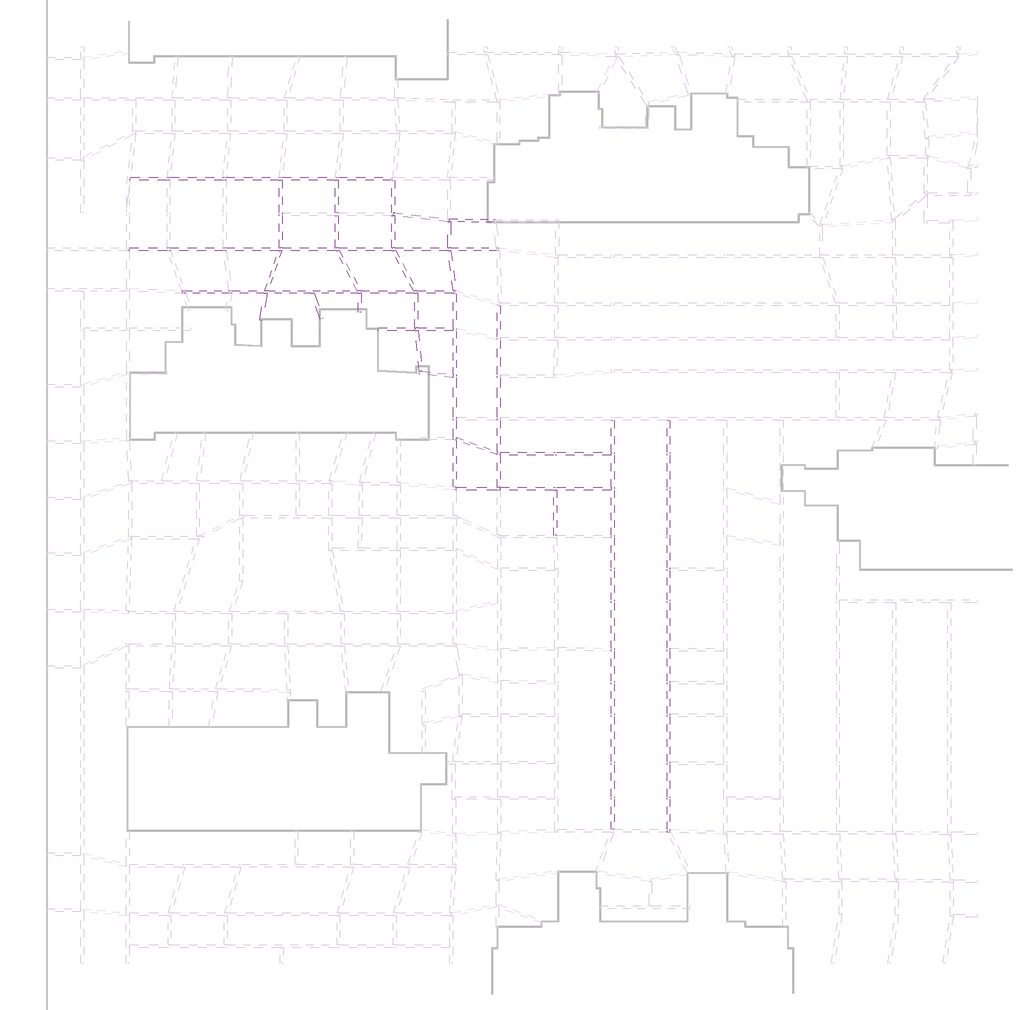
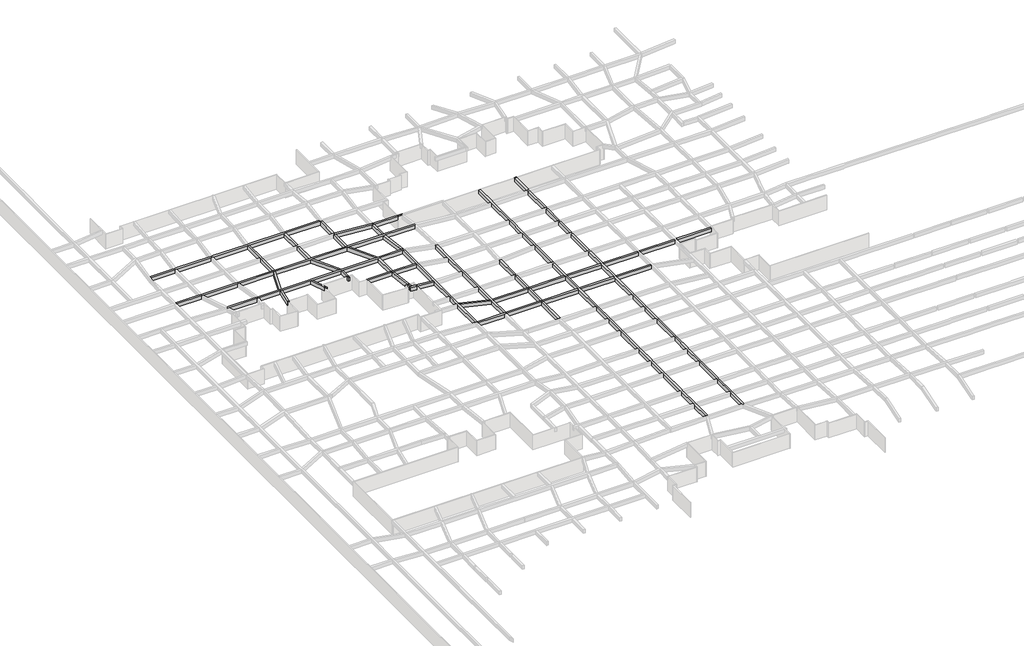
# One storey, part 27 of 45: 32 beams.
"""IFC4 building model written with IfcOpenShell, lengths in millimetres."""

from ifc_helpers import new_model, si_unit, frame, origin, place, context, project, spatial, polyline, outline, extrude, faceted_brep, element, save

model = new_model("IFC4")

# Units and contexts
model_context = context("Model", 3, world=origin())
ifc_project = project(units=[si_unit("LENGTHUNIT", "METRE", prefix="MILLI")], contexts=[model_context])

# Site, building, storey
site = spatial("IfcSite", under=ifc_project)
building = spatial("IfcBuilding", under=site)
storey = spatial("IfcBuildingStorey", under=building, Name="户型图", Elevation=0.0)

# Beams
placement = place(None, origin())
element("IfcBeam", 1, ObjectType="混凝土 - 矩形梁 : KL_beam", at=placement, inside=storey, context=model_context, shape_type="Brep", body=[
    faceted_brep([(-76574.0592951, 55456.2114264, 3300.0), (-76574.0592951, 55456.2114264, 2500.0), (-76974.0592951, 55456.2114264, 2500.0), (-76974.0592951, 55456.2114264, 3300.0), (-76574.0592951, 28384.5858537, 3300.0), (-76974.0592951, 28384.5858537, 3300.0), (-76974.0592951, 28384.5858537, 2500.0), (-76574.0592951, 28384.5858537, 2500.0), (-76974.0592951, 50864.7430833, 3300.0), (-76974.0592951, 50464.7430833, 3300.0), (-76974.0592951, 44242.2010773, 3300.0), (-76974.0592951, 43842.2010773, 3300.0), (-76974.0592951, 39470.5101546, 3300.0), (-76974.0592951, 39070.5101546, 3300.0), (-76974.0592951, 34954.5846853, 3300.0), (-76974.0592951, 34553.0567503, 3300.0), (-76574.0592951, 34571.3370449, 3300.0), (-76574.0592951, 34971.3370449, 3300.0), (-76574.0592951, 39070.5101546, 3300.0), (-76574.0592951, 39470.5101546, 3300.0), (-76574.0592951, 43842.2010773, 3300.0), (-76574.0592951, 44242.2010773, 3300.0), (-76574.0592951, 50450.070339, 3300.0), (-76574.0592951, 50850.070339, 3300.0), (-76974.0592951, 50864.7430833, 2500.0), (-76974.0592951, 50464.7430833, 2500.0), (-76974.0592951, 44242.2010773, 2500.0), (-76974.0592951, 43842.2010773, 2500.0), (-76974.0592951, 39470.5101546, 2500.0), (-76974.0592951, 39070.5101546, 2500.0), (-76974.0592951, 34954.5846853, 2500.0), (-76974.0592951, 34553.0567503, 2500.0), (-76574.0592951, 50850.070339, 2500.0), (-76574.0592951, 50450.070339, 2500.0), (-76574.0592951, 44242.2010773, 2500.0), (-76574.0592951, 43842.2010773, 2500.0), (-76574.0592951, 39470.5101546, 2500.0), (-76574.0592951, 39070.5101546, 2500.0), (-76574.0592951, 34971.3370449, 2500.0), (-76574.0592951, 34571.3370449, 2500.0)], [[[0, 1, 2, 3]], [[4, 5, 6, 7]], [[0, 3, 8, 9, 10, 11, 12, 13, 14, 15, 5, 4, 16, 17, 18, 19, 20, 21, 22, 23]], [[3, 2, 24, 25, 26, 27, 28, 29, 30, 31, 6, 5, 15, 14, 13, 12, 11, 10, 9, 8]], [[2, 1, 32, 33, 34, 35, 36, 37, 38, 39, 7, 6, 31, 30, 29, 28, 27, 26, 25, 24]], [[1, 0, 23, 22, 21, 20, 19, 18, 17, 16, 4, 7, 39, 38, 37, 36, 35, 34, 33, 32]]]),
    faceted_brep([(-76574.0592951, 27984.5858537, 3300.0), (-76974.0592951, 27984.5858537, 3300.0), (-76974.0592951, 23571.3370449, 3300.0), (-76974.0592951, 23171.3370449, 3300.0), (-76974.0592951, 18720.4464741, 3300.0), (-76974.0592951, 18320.4464741, 3300.0), (-76974.0592951, 12100.217385, 3300.0), (-76974.0592951, 11700.217385, 3300.0), (-76974.0592951, 7600.318112, 3300.0), (-76974.0592951, 7200.318112, 3300.0), (-76974.0592951, 3119.5822838, 3300.0), (-76974.0592951, 2719.5822838, 3300.0), (-76974.0592951, -3547.9984335, 3300.0), (-76974.0592951, -3948.0593648, 3300.0), (-76974.0592951, -8106.533538, 3300.0), (-76974.0592951, -8506.533538, 3300.0), (-76974.0592951, -12606.533538, 3300.0), (-76974.0592951, -13006.533538, 3300.0), (-76974.0592951, -19266.2432363, 3300.0), (-76974.0592951, -19666.2432363, 3300.0), (-76974.0592951, -24066.2432363, 3300.0), (-76974.0592951, -24466.2432363, 3300.0), (-76974.0592951, -28597.0413366, 3300.0), (-76574.0592951, -28597.0413366, 3300.0), (-76574.0592951, -24466.2432363, 3300.0), (-76574.0592951, -24066.2432363, 3300.0), (-76574.0592951, -19666.2432363, 3300.0), (-76574.0592951, -19266.2432363, 3300.0), (-76574.0592951, -13006.533538, 3300.0), (-76574.0592951, -12606.533538, 3300.0), (-76574.0592951, -8506.533538, 3300.0), (-76574.0592951, -8106.533538, 3300.0), (-76574.0592951, -3951.5199121, 3300.0), (-76574.0592951, -3551.5199121, 3300.0), (-76574.0592951, 2719.5822838, 3300.0), (-76574.0592951, 3119.5822838, 3300.0), (-76574.0592951, 7200.318112, 3300.0), (-76574.0592951, 7600.318112, 3300.0), (-76574.0592951, 11700.217385, 3300.0), (-76574.0592951, 12100.217385, 3300.0), (-76574.0592951, 18320.4464741, 3300.0), (-76574.0592951, 18720.4464741, 3300.0), (-76574.0592951, 23171.3370449, 3300.0), (-76574.0592951, 23571.3370449, 3300.0), (-76974.0592951, 27984.5858537, 2500.0), (-76974.0592951, 23571.3370449, 2500.0), (-76974.0592951, 23171.3370449, 2500.0), (-76974.0592951, 18720.4464741, 2500.0), (-76974.0592951, 18320.4464741, 2500.0), (-76974.0592951, 12100.217385, 2500.0), (-76974.0592951, 11700.217385, 2500.0), (-76974.0592951, 7600.318112, 2500.0), (-76974.0592951, 7200.318112, 2500.0), (-76974.0592951, 3119.5822838, 2500.0), (-76974.0592951, 2719.5822838, 2500.0), (-76974.0592951, -3547.9984335, 2500.0), (-76974.0592951, -3948.0593648, 2500.0), (-76974.0592951, -8106.533538, 2500.0), (-76974.0592951, -8506.533538, 2500.0), (-76974.0592951, -12606.533538, 2500.0), (-76974.0592951, -13006.533538, 2500.0), (-76974.0592951, -19266.2432363, 2500.0), (-76974.0592951, -19666.2432363, 2500.0), (-76974.0592951, -24066.2432363, 2500.0), (-76974.0592951, -24466.2432363, 2500.0), (-76974.0592951, -28597.0413366, 2500.0), (-76574.0592951, 27984.5858537, 2500.0), (-76574.0592951, 23571.3370449, 2500.0), (-76574.0592951, 23171.3370449, 2500.0), (-76574.0592951, 18720.4464741, 2500.0), (-76574.0592951, 18320.4464741, 2500.0), (-76574.0592951, 12100.217385, 2500.0), (-76574.0592951, 11700.217385, 2500.0), (-76574.0592951, 7600.318112, 2500.0), (-76574.0592951, 7200.318112, 2500.0), (-76574.0592951, 3119.5822838, 2500.0), (-76574.0592951, 2719.5822838, 2500.0), (-76574.0592951, -3551.5199121, 2500.0), (-76574.0592951, -3951.5199121, 2500.0), (-76574.0592951, -8106.533538, 2500.0), (-76574.0592951, -8506.533538, 2500.0), (-76574.0592951, -12606.533538, 2500.0), (-76574.0592951, -13006.533538, 2500.0), (-76574.0592951, -19266.2432363, 2500.0), (-76574.0592951, -19666.2432363, 2500.0), (-76574.0592951, -24066.2432363, 2500.0), (-76574.0592951, -24466.2432363, 2500.0), (-76574.0592951, -28597.0413366, 2500.0)], [[[0, 1, 2, 3, 4, 5, 6, 7, 8, 9, 10, 11, 12, 13, 14, 15, 16, 17, 18, 19, 20, 21, 22, 23, 24, 25, 26, 27, 28, 29, 30, 31, 32, 33, 34, 35, 36, 37, 38, 39, 40, 41, 42, 43]], [[1, 44, 45, 46, 47, 48, 49, 50, 51, 52, 53, 54, 55, 56, 57, 58, 59, 60, 61, 62, 63, 64, 65, 22, 21, 20, 19, 18, 17, 16, 15, 14, 13, 12, 11, 10, 9, 8, 7, 6, 5, 4, 3, 2]], [[44, 66, 67, 68, 69, 70, 71, 72, 73, 74, 75, 76, 77, 78, 79, 80, 81, 82, 83, 84, 85, 86, 87, 65, 64, 63, 62, 61, 60, 59, 58, 57, 56, 55, 54, 53, 52, 51, 50, 49, 48, 47, 46, 45]], [[66, 0, 43, 42, 41, 40, 39, 38, 37, 36, 35, 34, 33, 32, 31, 30, 29, 28, 27, 26, 25, 24, 23, 87, 86, 85, 84, 83, 82, 81, 80, 79, 78, 77, 76, 75, 74, 73, 72, 71, 70, 69, 68, 67]], [[1, 0, 66, 44]], [[23, 22, 65, 87]]]),
])
element("IfcBeam", 2, ObjectType="混凝土 - 矩形梁 : KL_beam", at=placement, inside=storey, context=model_context, shape_type="Brep", body=[
    faceted_brep([(-68859.410716, 55506.2431184, 3300.0), (-68859.410716, 55506.2431184, 2500.0), (-69259.410716, 55506.2431184, 2500.0), (-69259.410716, 55506.2431184, 3300.0), (-68859.410716, 50850.070339, 3300.0), (-69259.410716, 50850.070339, 3300.0), (-69259.410716, 50850.070339, 2500.0), (-68859.410716, 50850.070339, 2500.0)], [[[0, 1, 2, 3]], [[4, 5, 6, 7]], [[0, 3, 5, 4]], [[3, 2, 6, 5]], [[2, 1, 7, 6]], [[1, 0, 4, 7]]]),
    faceted_brep([(-68859.410716, 27984.5858537, 3300.0), (-69259.410716, 27984.5858537, 3300.0), (-69259.410716, 23571.3370449, 3300.0), (-69259.410716, 23171.3370449, 3300.0), (-69259.410716, 18720.4464741, 3300.0), (-69259.410716, 18320.4464741, 3300.0), (-69259.410716, 12100.217385, 3300.0), (-69259.410716, 11700.217385, 3300.0), (-69259.410716, 7600.318112, 3300.0), (-69259.410716, 7200.318112, 3300.0), (-69259.410716, 3119.5822838, 3300.0), (-69259.410716, 2719.5822838, 3300.0), (-69259.410716, -3551.5199121, 3300.0), (-69259.410716, -3951.5199121, 3300.0), (-69259.410716, -8106.533538, 3300.0), (-69259.410716, -8506.533538, 3300.0), (-69259.410716, -12606.533538, 3300.0), (-69259.410716, -13006.533538, 3300.0), (-69259.410716, -19266.2432363, 3300.0), (-69259.410716, -19666.2432363, 3300.0), (-69259.410716, -24066.2432363, 3300.0), (-69259.410716, -24466.2432363, 3300.0), (-69259.410716, -28597.0413366, 3300.0), (-69259.410716, -28997.0413366, 3300.0), (-69183.9947177, -28997.0413366, 3300.0), (-69062.8285047, -28997.0413366, 3300.0), (-68859.410716, -28997.0413366, 3300.0), (-68859.410716, -28603.762064, 3300.0), (-68859.410716, -24466.2432363, 3300.0), (-68859.410716, -24066.2432363, 3300.0), (-68859.410716, -19666.2432363, 3300.0), (-68859.410716, -19266.2432363, 3300.0), (-68859.410716, -13006.533538, 3300.0), (-68859.410716, -12606.533538, 3300.0), (-68859.410716, -8506.533538, 3300.0), (-68859.410716, -8106.533538, 3300.0), (-68859.410716, -3951.5199121, 3300.0), (-68859.410716, -3551.5199121, 3300.0), (-68859.410716, 2719.5822838, 3300.0), (-68859.410716, 3119.5822838, 3300.0), (-68859.410716, 7200.318112, 3300.0), (-68859.410716, 7600.318112, 3300.0), (-68859.410716, 11700.217385, 3300.0), (-68859.410716, 12100.217385, 3300.0), (-68859.410716, 18320.4464741, 3300.0), (-68859.410716, 18720.4464741, 3300.0), (-68859.410716, 23171.3370449, 3300.0), (-68859.410716, 23571.3370449, 3300.0), (-69259.410716, 27984.5858537, 2500.0), (-69259.410716, 23571.3370449, 2500.0), (-69259.410716, 23171.3370449, 2500.0), (-69259.410716, 18720.4464741, 2500.0), (-69259.410716, 18320.4464741, 2500.0), (-69259.410716, 12100.217385, 2500.0), (-69259.410716, 11700.217385, 2500.0), (-69259.410716, 7600.318112, 2500.0), (-69259.410716, 7200.318112, 2500.0), (-69259.410716, 3119.5822838, 2500.0), (-69259.410716, 2719.5822838, 2500.0), (-69259.410716, -3551.5199121, 2500.0), (-69259.410716, -3951.5199121, 2500.0), (-69259.410716, -8106.533538, 2500.0), (-69259.410716, -8506.533538, 2500.0), (-69259.410716, -12606.533538, 2500.0), (-69259.410716, -13006.533538, 2500.0), (-69259.410716, -19266.2432363, 2500.0), (-69259.410716, -19666.2432363, 2500.0), (-69259.410716, -24066.2432363, 2500.0), (-69259.410716, -24466.2432363, 2500.0), (-69259.410716, -28597.0413366, 2500.0), (-69259.410716, -28997.0413366, 2500.0), (-68859.410716, 27984.5858537, 2500.0), (-68859.410716, 23571.3370449, 2500.0), (-68859.410716, 23171.3370449, 2500.0), (-68859.410716, 18720.4464741, 2500.0), (-68859.410716, 18320.4464741, 2500.0), (-68859.410716, 12100.217385, 2500.0), (-68859.410716, 11700.217385, 2500.0), (-68859.410716, 7600.318112, 2500.0), (-68859.410716, 7200.318112, 2500.0), (-68859.410716, 3119.5822838, 2500.0), (-68859.410716, 2719.5822838, 2500.0), (-68859.410716, -3551.5199121, 2500.0), (-68859.410716, -3951.5199121, 2500.0), (-68859.410716, -8106.533538, 2500.0), (-68859.410716, -8506.533538, 2500.0), (-68859.410716, -12606.533538, 2500.0), (-68859.410716, -13006.533538, 2500.0), (-68859.410716, -19266.2432363, 2500.0), (-68859.410716, -19666.2432363, 2500.0), (-68859.410716, -24066.2432363, 2500.0), (-68859.410716, -24466.2432363, 2500.0), (-68859.410716, -28603.762064, 2500.0), (-68859.410716, -28997.0413366, 2500.0), (-69062.8285047, -28997.0413366, 2500.0), (-69183.9947177, -28997.0413366, 2500.0)], [[[0, 1, 2, 3, 4, 5, 6, 7, 8, 9, 10, 11, 12, 13, 14, 15, 16, 17, 18, 19, 20, 21, 22, 23, 24, 25, 26, 27, 28, 29, 30, 31, 32, 33, 34, 35, 36, 37, 38, 39, 40, 41, 42, 43, 44, 45, 46, 47]], [[1, 48, 49, 50, 51, 52, 53, 54, 55, 56, 57, 58, 59, 60, 61, 62, 63, 64, 65, 66, 67, 68, 69, 70, 23, 22, 21, 20, 19, 18, 17, 16, 15, 14, 13, 12, 11, 10, 9, 8, 7, 6, 5, 4, 3, 2]], [[48, 71, 72, 73, 74, 75, 76, 77, 78, 79, 80, 81, 82, 83, 84, 85, 86, 87, 88, 89, 90, 91, 92, 93, 94, 95, 70, 69, 68, 67, 66, 65, 64, 63, 62, 61, 60, 59, 58, 57, 56, 55, 54, 53, 52, 51, 50, 49]], [[71, 0, 47, 46, 45, 44, 43, 42, 41, 40, 39, 38, 37, 36, 35, 34, 33, 32, 31, 30, 29, 28, 27, 26, 93, 92, 91, 90, 89, 88, 87, 86, 85, 84, 83, 82, 81, 80, 79, 78, 77, 76, 75, 74, 73, 72]], [[1, 0, 71, 48]], [[26, 25, 24, 23, 70, 95, 94, 93]]]),
    faceted_brep([(-68859.410716, 28384.5858537, 3300.0), (-69259.410716, 28384.5858537, 3300.0), (-69259.410716, 28384.5858537, 2500.0), (-68859.410716, 28384.5858537, 2500.0), (-68859.410716, 34571.3370449, 3300.0), (-69259.410716, 34571.3370449, 3300.0), (-69259.410716, 34571.3370449, 2500.0), (-68859.410716, 34571.3370449, 2500.0)], [[[0, 1, 2, 3]], [[1, 0, 4, 5]], [[2, 1, 5, 6]], [[3, 2, 6, 7]], [[0, 3, 7, 4]], [[5, 4, 7, 6]]]),
    faceted_brep([(-68859.410716, 34971.3370449, 3300.0), (-69259.410716, 34971.3370449, 3300.0), (-69259.410716, 34971.3370449, 2500.0), (-68859.410716, 34971.3370449, 2500.0), (-68859.410716, 39070.5101546, 3300.0), (-69259.410716, 39070.5101546, 3300.0), (-69259.410716, 39070.5101546, 2500.0), (-68859.410716, 39070.5101546, 2500.0)], [[[0, 1, 2, 3]], [[1, 0, 4, 5]], [[2, 1, 5, 6]], [[3, 2, 6, 7]], [[0, 3, 7, 4]], [[5, 4, 7, 6]]]),
    faceted_brep([(-68859.410716, 39470.5101546, 3300.0), (-69259.410716, 39470.5101546, 3300.0), (-69259.410716, 39470.5101546, 2500.0), (-68859.410716, 39470.5101546, 2500.0), (-68859.410716, 43842.2010773, 3300.0), (-69259.410716, 43842.2010773, 3300.0), (-69259.410716, 43842.2010773, 2500.0), (-68859.410716, 43842.2010773, 2500.0)], [[[0, 1, 2, 3]], [[1, 0, 4, 5]], [[2, 1, 5, 6]], [[3, 2, 6, 7]], [[0, 3, 7, 4]], [[5, 4, 7, 6]]]),
    faceted_brep([(-68859.410716, 44242.2010773, 3300.0), (-69259.410716, 44242.2010773, 3300.0), (-69259.410716, 44242.2010773, 2500.0), (-68859.410716, 44242.2010773, 2500.0), (-68859.410716, 50450.070339, 3300.0), (-69259.410716, 50450.070339, 3300.0), (-69259.410716, 50450.070339, 2500.0), (-68859.410716, 50450.070339, 2500.0)], [[[0, 1, 2, 3]], [[1, 0, 4, 5]], [[2, 1, 5, 6]], [[3, 2, 6, 7]], [[0, 3, 7, 4]], [[5, 4, 7, 6]]]),
])
element("IfcBeam", 3, ObjectType="混凝土 - 矩形梁 : KL_beam", at=placement, inside=storey, context=model_context, shape_type="Brep", body=[
    faceted_brep([(-107354.1744669, 61170.3096597, 3300.0), (-107354.1744669, 61570.3096597, 3300.0), (-114692.5916069, 61570.3096597, 3300.0), (-115094.7622577, 61570.3096597, 3300.0), (-122492.6084803, 61570.3096597, 3300.0), (-122894.779131, 61570.3096597, 3300.0), (-130266.1701137, 61570.3096597, 3300.0), (-130292.5916069, 61570.3096597, 3300.0), (-130694.7622577, 61570.3096597, 3300.0), (-137992.6084803, 61570.3096597, 3300.0), (-138394.779131, 61570.3096597, 3300.0), (-143507.3765183, 61570.3096597, 3300.0), (-143556.4903427, 61170.3096597, 3300.0), (-138430.1531976, 61170.3096597, 3300.0), (-138030.1531976, 61170.3096597, 3300.0), (-130666.1701137, 61170.3096597, 3300.0), (-130266.1701137, 61170.3096597, 3300.0), (-122902.1870297, 61170.3096597, 3300.0), (-122502.1870297, 61170.3096597, 3300.0), (-115128.2029549, 61170.3096597, 3300.0), (-114728.2029549, 61170.3096597, 3300.0), (-107354.1744669, 61170.3096597, 2500.0), (-143556.4903427, 61170.3096597, 2500.0), (-138430.1531976, 61170.3096597, 2500.0), (-138030.1531976, 61170.3096597, 2500.0), (-130666.1701137, 61170.3096597, 2500.0), (-130266.1701137, 61170.3096597, 2500.0), (-122902.1870297, 61170.3096597, 2500.0), (-122502.1870297, 61170.3096597, 2500.0), (-115128.2029549, 61170.3096597, 2500.0), (-114728.2029549, 61170.3096597, 2500.0), (-107354.1744669, 61570.3096597, 2500.0), (-143507.3765183, 61570.3096597, 2500.0), (-138394.779131, 61570.3096597, 2500.0), (-137992.6084803, 61570.3096597, 2500.0), (-130694.7622577, 61570.3096597, 2500.0), (-130292.5916069, 61570.3096597, 2500.0), (-130266.1701137, 61570.3096597, 2500.0), (-122894.779131, 61570.3096597, 2500.0), (-122492.6084803, 61570.3096597, 2500.0), (-115094.7622577, 61570.3096597, 2500.0), (-114692.5916069, 61570.3096597, 2500.0)], [[[0, 1, 2, 3, 4, 5, 6, 7, 8, 9, 10, 11, 12, 13, 14, 15, 16, 17, 18, 19, 20]], [[21, 0, 20, 19, 18, 17, 16, 15, 14, 13, 12, 22, 23, 24, 25, 26, 27, 28, 29, 30]], [[31, 21, 30, 29, 28, 27, 26, 25, 24, 23, 22, 32, 33, 34, 35, 36, 37, 38, 39, 40, 41]], [[1, 31, 41, 40, 39, 38, 37, 36, 35, 34, 33, 32, 11, 10, 9, 8, 7, 6, 5, 4, 3, 2]], [[1, 0, 21, 31]], [[12, 11, 32, 22]]]),
])
element("IfcBeam", 4, ObjectType="混凝土 - 矩形梁 : KL_beam", at=placement, inside=storey, context=model_context, shape_type="SweptSolid", body=[
    extrude(outline(polyline([(-106954.1744669, 56704.7417755), (-107354.1744669, 56704.7417755), (-107354.1744669, 61170.3096597), (-106954.1744669, 61170.3096597), (-106954.1744669, 56704.7417755)])), frame((0.0, 0.0, 2500.0), z_axis=(0.0, 0.0, 1.0), x_axis=(1.0, 0.0, 0.0)), (0.0, 0.0, 1.0), 800.0),
])
element("IfcBeam", 5, ObjectType="混凝土 - 矩形梁 : KL_beam", at=placement, inside=storey, context=model_context, shape_type="SweptSolid", body=[
    extrude(outline(polyline([(-115128.2029549, 61170.3096597), (-114728.2029549, 61170.3096597), (-114728.2029549, 56692.8612022), (-115128.2029549, 56692.8612022), (-115128.2029549, 61170.3096597)])), frame((0.0, 0.0, 2500.0), z_axis=(0.0, 0.0, 1.0), x_axis=(1.0, 0.0, 0.0)), (0.0, 0.0, 1.0), 800.0),
])
element("IfcBeam", 6, ObjectType="混凝土 - 矩形梁 : KL_beam", at=placement, inside=storey, context=model_context, shape_type="Brep", body=[
    faceted_brep([(-122502.1870297, 61170.3096597, 3300.0), (-122902.1870297, 61170.3096597, 3300.0), (-122902.1870297, 56692.8612022, 3300.0), (-122902.1870297, 56292.8612022, 3300.0), (-122902.1870297, 51854.9299556, 3300.0), (-122502.1870297, 51854.9299556, 3300.0), (-122502.1870297, 56292.8612022, 3300.0), (-122502.1870297, 56692.8612022, 3300.0), (-122502.1870297, 61170.3096597, 2500.0), (-122502.1870297, 51854.9299556, 2500.0), (-122502.1870297, 56292.8612022, 2500.0), (-122502.1870297, 56692.8612022, 2500.0), (-122902.1870297, 61170.3096597, 2500.0), (-122902.1870297, 51854.9299556, 2500.0), (-122902.1870297, 56292.8612022, 2500.0), (-122902.1870297, 56692.8612022, 2500.0)], [[[0, 1, 2, 3, 4, 5, 6, 7]], [[8, 0, 7, 6, 5, 9, 10, 11]], [[12, 8, 11, 10, 9, 13, 14, 15]], [[1, 12, 15, 14, 13, 4, 3, 2]], [[1, 0, 8, 12]], [[5, 4, 13, 9]]]),
])
element("IfcBeam", 7, ObjectType="混凝土 - 矩形梁 : KL_beam", at=placement, inside=storey, context=model_context, shape_type="Brep", body=[
    faceted_brep([(-92641.4119842, 51454.9299556, 3300.0), (-92616.9469361, 51854.9299556, 3300.0), (-92859.0655317, 51854.9299556, 3300.0), (-99175.6871975, 51854.9299556, 3300.0), (-99575.6871975, 51854.9299556, 3300.0), (-106954.1744669, 51854.9299556, 3300.0), (-107354.1744669, 51854.9299556, 3300.0), (-114728.2029549, 51854.9299556, 3300.0), (-115128.2029549, 51854.9299556, 3300.0), (-122502.1870297, 51854.9299556, 3300.0), (-122902.1870297, 51854.9299556, 3300.0), (-130266.1701137, 51854.9299556, 3300.0), (-130666.1701137, 51854.9299556, 3300.0), (-138030.1531976, 51854.9299556, 3300.0), (-138430.1531976, 51854.9299556, 3300.0), (-143629.1794601, 51854.9299556, 3300.0), (-143629.1794601, 51454.9299556, 3300.0), (-138371.532439, 51454.9299556, 3300.0), (-137947.2933339, 51454.9299556, 3300.0), (-130640.0234877, 51454.9299556, 3300.0), (-130236.0924587, 51454.9299556, 3300.0), (-122982.6420599, 51454.9299556, 3300.0), (-122559.5937874, 51454.9299556, 3300.0), (-115048.1275024, 51454.9299556, 3300.0), (-114595.0994822, 51454.9299556, 3300.0), (-107274.1222264, 51454.9299556, 3300.0), (-106821.0942061, 51454.9299556, 3300.0), (-99552.2294815, 51454.9299556, 3300.0), (-99149.1194947, 51454.9299556, 3300.0), (-92822.5012905, 51454.9299556, 3300.0), (-92641.4119842, 51454.9299556, 2500.0), (-143629.1794601, 51454.9299556, 2500.0), (-138371.532439, 51454.9299556, 2500.0), (-137947.2933339, 51454.9299556, 2500.0), (-130640.0234877, 51454.9299556, 2500.0), (-130236.0924587, 51454.9299556, 2500.0), (-122982.6420599, 51454.9299556, 2500.0), (-122559.5937874, 51454.9299556, 2500.0), (-115048.1275024, 51454.9299556, 2500.0), (-114595.0994822, 51454.9299556, 2500.0), (-107274.1222264, 51454.9299556, 2500.0), (-106821.0942061, 51454.9299556, 2500.0), (-99552.2294815, 51454.9299556, 2500.0), (-99149.1194947, 51454.9299556, 2500.0), (-92822.5012905, 51454.9299556, 2500.0), (-92616.9469361, 51854.9299556, 2500.0), (-143629.1794601, 51854.9299556, 2500.0), (-138430.1531976, 51854.9299556, 2500.0), (-138030.1531976, 51854.9299556, 2500.0), (-130666.1701137, 51854.9299556, 2500.0), (-130266.1701137, 51854.9299556, 2500.0), (-122902.1870297, 51854.9299556, 2500.0), (-122502.1870297, 51854.9299556, 2500.0), (-115128.2029549, 51854.9299556, 2500.0), (-114728.2029549, 51854.9299556, 2500.0), (-107354.1744669, 51854.9299556, 2500.0), (-106954.1744669, 51854.9299556, 2500.0), (-99575.6871975, 51854.9299556, 2500.0), (-99175.6871975, 51854.9299556, 2500.0), (-92859.0655317, 51854.9299556, 2500.0)], [[[0, 1, 2, 3, 4, 5, 6, 7, 8, 9, 10, 11, 12, 13, 14, 15, 16, 17, 18, 19, 20, 21, 22, 23, 24, 25, 26, 27, 28, 29]], [[30, 0, 29, 28, 27, 26, 25, 24, 23, 22, 21, 20, 19, 18, 17, 16, 31, 32, 33, 34, 35, 36, 37, 38, 39, 40, 41, 42, 43, 44]], [[45, 30, 44, 43, 42, 41, 40, 39, 38, 37, 36, 35, 34, 33, 32, 31, 46, 47, 48, 49, 50, 51, 52, 53, 54, 55, 56, 57, 58, 59]], [[1, 45, 59, 58, 57, 56, 55, 54, 53, 52, 51, 50, 49, 48, 47, 46, 15, 14, 13, 12, 11, 10, 9, 8, 7, 6, 5, 4, 3, 2]], [[16, 15, 46, 31]], [[1, 0, 30, 45]]]),
])
element("IfcBeam", 8, ObjectType="混凝土 - 矩形梁 : KL_beam", at=placement, inside=storey, context=model_context, shape_type="Brep", body=[
    faceted_brep([(-99387.6207865, 55458.4802016, 3300.0), (-99175.6871975, 55454.7808871, 3300.0), (-93350.7020276, 55353.1053927, 3300.0), (-93398.6713053, 55694.4245387, 3300.0), (-93021.5786579, 55747.4214542, 3300.0), (-99231.1820439, 55855.8104845, 3300.0), (-99363.3334842, 55858.1171964, 3300.0), (-93021.5786579, 55747.4214542, 2500.0), (-99231.1820439, 55855.8104845, 2500.0), (-99363.3334842, 55858.1171964, 2500.0), (-93398.6713053, 55694.4245387, 2500.0), (-93350.7020276, 55353.1053927, 2500.0), (-99175.6871975, 55454.7808871, 2500.0), (-99387.6207865, 55458.4802016, 2500.0)], [[[0, 1, 2, 3, 4, 5, 6]], [[6, 5, 4, 7, 8, 9]], [[9, 8, 7, 10, 11, 12, 13]], [[2, 1, 0, 13, 12, 11]], [[10, 3, 2, 11]], [[3, 10, 7, 4]], [[0, 6, 9, 13]]]),
])
element("IfcBeam", 9, ObjectType="混凝土 - 矩形梁 : KL_beam", at=placement, inside=storey, context=model_context, shape_type="Brep", body=[
    faceted_brep([(-99387.6207865, 55458.4802016, 3300.0), (-99363.3334842, 55858.1171964, 3300.0), (-99631.1820439, 55886.0592094, 3300.0), (-107154.3480617, 56670.8773262, 3300.0), (-107154.3480617, 56292.8612022, 3300.0), (-107385.8902631, 56292.8612022, 3300.0), (-107354.1744669, 56289.5526042, 3300.0), (-106954.1744669, 56247.8245278, 3300.0), (-99575.6871975, 55478.0993256, 3300.0), (-99363.3334842, 55858.1171964, 2500.0), (-99631.1820439, 55886.0592094, 2500.0), (-107154.3480617, 56670.8773262, 2500.0), (-99387.6207865, 55458.4802016, 2500.0), (-99575.6871975, 55478.0993256, 2500.0), (-106954.1744669, 56247.8245278, 2500.0), (-107354.1744669, 56289.5526042, 2500.0), (-107385.8902631, 56292.8612022, 2500.0), (-107154.3480617, 56292.8612022, 2500.0)], [[[0, 1, 2, 3, 4, 5, 6, 7, 8]], [[1, 9, 10, 11, 3, 2]], [[9, 12, 13, 14, 15, 16, 17, 11, 10]], [[12, 0, 8, 7, 6, 5, 16, 15, 14, 13]], [[0, 12, 9, 1]], [[4, 17, 16, 5]], [[17, 4, 3, 11]]]),
])
element("IfcBeam", 10, ObjectType="混凝土 - 矩形梁 : KL_beam", at=placement, inside=storey, context=model_context, shape_type="Brep", body=[
    faceted_brep([(-99575.6871975, 51854.9299556, 3300.0), (-99175.6871975, 51854.9299556, 3300.0), (-99175.6871975, 55454.7808871, 3300.0), (-99231.1820439, 55455.7495532, 3300.0), (-99387.6207865, 55458.4802016, 3300.0), (-99575.6871975, 55478.0993256, 3300.0), (-99575.6871975, 51854.9299556, 2500.0), (-99575.6871975, 55478.0993256, 2500.0), (-99175.6871975, 51854.9299556, 2500.0), (-99387.6207865, 55458.4802016, 2500.0), (-99231.1820439, 55455.7495532, 2500.0), (-99175.6871975, 55454.7808871, 2500.0)], [[[0, 1, 2, 3, 4, 5]], [[6, 0, 5, 7]], [[8, 6, 7, 9, 10, 11]], [[1, 8, 11, 2]], [[1, 0, 6, 8]], [[5, 4, 9, 7]], [[2, 11, 10, 9, 4, 3]]]),
])
element("IfcBeam", 11, ObjectType="混凝土 - 矩形梁 : KL_beam", at=placement, inside=storey, context=model_context, shape_type="SweptSolid", body=[
    extrude(outline(polyline([(-106954.1744669, 51854.9299556), (-107354.1744669, 51854.9299556), (-107354.1744669, 56289.5526042), (-106954.1744669, 56247.8245278), (-106954.1744669, 51854.9299556)])), frame((0.0, 0.0, 2500.0), z_axis=(0.0, 0.0, 1.0), x_axis=(1.0, 0.0, 0.0)), (0.0, 0.0, 1.0), 800.0),
])
element("IfcBeam", 12, ObjectType="混凝土 - 矩形梁 : KL_beam", at=placement, inside=storey, context=model_context, shape_type="SweptSolid", body=[
    extrude(outline(polyline([(-115128.2029549, 56292.8612022), (-114728.2029549, 56292.8612022), (-114728.2029549, 51854.9299556), (-115128.2029549, 51854.9299556), (-115128.2029549, 56292.8612022)])), frame((0.0, 0.0, 2500.0), z_axis=(0.0, 0.0, 1.0), x_axis=(1.0, 0.0, 0.0)), (0.0, 0.0, 1.0), 800.0),
])
element("IfcBeam", 13, ObjectType="混凝土 - 矩形梁 : KL_beam", at=placement, inside=storey, context=model_context, shape_type="Brep", body=[
    faceted_brep([(-98660.8661571, 45524.6770642, 3300.0), (-98608.2051581, 45924.6770642, 3300.0), (-98861.2712603, 45924.6770642, 3300.0), (-103880.6065843, 45924.6770642, 3300.0), (-104333.6346046, 45924.6770642, 3300.0), (-111654.6118603, 45924.6770642, 3300.0), (-112107.6398806, 45924.6770642, 3300.0), (-124463.8125664, 45924.6770642, 3300.0), (-124886.8608389, 45924.6770642, 3300.0), (-129458.8661012, 45924.6770642, 3300.0), (-129862.7971302, 45924.6770642, 3300.0), (-135993.089329, 45924.6770642, 3300.0), (-136417.3284341, 45924.6770642, 3300.0), (-136275.9819863, 45524.6770642, 3300.0), (-135852.1282857, 45524.6770642, 3300.0), (-129871.1577722, 45524.6770642, 3300.0), (-129464.9871274, 45524.6770642, 3300.0), (-124982.5529438, 45524.6770642, 3300.0), (-124576.382299, 45524.6770642, 3300.0), (-118475.9819863, 45524.6770642, 3300.0), (-118051.7428811, 45524.6770642, 3300.0), (-111974.7839841, 45524.6770642, 3300.0), (-111574.7839841, 45524.6770642, 3300.0), (-104134.5356576, 45524.6770642, 3300.0), (-103734.5356576, 45524.6770642, 3300.0), (-98834.5356576, 45524.6770642, 3300.0), (-98660.8661571, 45524.6770642, 2500.0), (-136275.9819863, 45524.6770642, 2500.0), (-135852.1282857, 45524.6770642, 2500.0), (-129871.1577722, 45524.6770642, 2500.0), (-129464.9871274, 45524.6770642, 2500.0), (-124982.5529438, 45524.6770642, 2500.0), (-124576.382299, 45524.6770642, 2500.0), (-118475.9819863, 45524.6770642, 2500.0), (-118051.7428811, 45524.6770642, 2500.0), (-111974.7839841, 45524.6770642, 2500.0), (-111574.7839841, 45524.6770642, 2500.0), (-104134.5356576, 45524.6770642, 2500.0), (-103734.5356576, 45524.6770642, 2500.0), (-98834.5356576, 45524.6770642, 2500.0), (-98608.2051581, 45924.6770642, 2500.0), (-136417.3284341, 45924.6770642, 2500.0), (-135993.089329, 45924.6770642, 2500.0), (-129862.7971302, 45924.6770642, 2500.0), (-129458.8661012, 45924.6770642, 2500.0), (-124886.8608389, 45924.6770642, 2500.0), (-124463.8125664, 45924.6770642, 2500.0), (-112107.6398806, 45924.6770642, 2500.0), (-111654.6118603, 45924.6770642, 2500.0), (-104333.6346046, 45924.6770642, 2500.0), (-103880.6065843, 45924.6770642, 2500.0), (-98861.2712603, 45924.6770642, 2500.0)], [[[0, 1, 2, 3, 4, 5, 6, 7, 8, 9, 10, 11, 12, 13, 14, 15, 16, 17, 18, 19, 20, 21, 22, 23, 24, 25]], [[26, 0, 25, 24, 23, 22, 21, 20, 19, 18, 17, 16, 15, 14, 13, 27, 28, 29, 30, 31, 32, 33, 34, 35, 36, 37, 38, 39]], [[40, 26, 39, 38, 37, 36, 35, 34, 33, 32, 31, 30, 29, 28, 27, 41, 42, 43, 44, 45, 46, 47, 48, 49, 50, 51]], [[1, 40, 51, 50, 49, 48, 47, 46, 45, 44, 43, 42, 41, 12, 11, 10, 9, 8, 7, 6, 5, 4, 3, 2]], [[1, 0, 26, 40]], [[13, 12, 41, 27]]]),
])
element("IfcBeam", 14, ObjectType="混凝土 - 矩形梁 : KL_beam", at=placement, inside=storey, context=model_context, shape_type="SweptSolid", body=[
    extrude(outline(polyline([(-99552.2294815, 51454.9299556), (-99149.1194947, 51454.9299556), (-98452.964117, 45883.0803526), (-98608.2051581, 45924.6770642), (-98861.2712603, 45924.6770642), (-99552.2294815, 51454.9299556)])), frame((0.0, 0.0, 2500.0), z_axis=(0.0, 0.0, 1.0), x_axis=(1.0, 0.0, 0.0)), (0.0, 0.0, 1.0), 800.0),
])
element("IfcBeam", 15, ObjectType="混凝土 - 矩形梁 : KL_beam", at=placement, inside=storey, context=model_context, shape_type="SweptSolid", body=[
    extrude(outline(polyline([(-107274.1222264, 51454.9299556), (-106821.0942061, 51454.9299556), (-103880.6065843, 45924.6770642), (-104333.6346046, 45924.6770642), (-107274.1222264, 51454.9299556)])), frame((0.0, 0.0, 2500.0), z_axis=(0.0, 0.0, 1.0), x_axis=(1.0, 0.0, 0.0)), (0.0, 0.0, 1.0), 800.0),
])
element("IfcBeam", 16, ObjectType="混凝土 - 矩形梁 : KL_beam", at=placement, inside=storey, context=model_context, shape_type="SweptSolid", body=[
    extrude(outline(polyline([(-115048.1275024, 51454.9299556), (-114595.0994822, 51454.9299556), (-111654.6118603, 45924.6770642), (-112107.6398806, 45924.6770642), (-115048.1275024, 51454.9299556)])), frame((0.0, 0.0, 2500.0), z_axis=(0.0, 0.0, 1.0), x_axis=(1.0, 0.0, 0.0)), (0.0, 0.0, 1.0), 800.0),
])
element("IfcBeam", 17, ObjectType="混凝土 - 矩形梁 : KL_beam", at=placement, inside=storey, context=model_context, shape_type="SweptSolid", body=[
    extrude(outline(polyline([(-122982.6420599, 51454.9299556), (-122559.5937874, 51454.9299556), (-124463.8125664, 45924.6770642), (-124886.8608389, 45924.6770642), (-122982.6420599, 51454.9299556)])), frame((0.0, 0.0, 2500.0), z_axis=(0.0, 0.0, 1.0), x_axis=(1.0, 0.0, 0.0)), (0.0, 0.0, 1.0), 800.0),
])
element("IfcBeam", 18, ObjectType="混凝土 - 矩形梁 : KL_beam", at=placement, inside=storey, context=model_context, shape_type="Brep", body=[
    faceted_brep([(-98430.038157, 18720.4464741, 3300.0), (-98447.5025342, 18320.4464741, 3300.0), (-98434.5356576, 18320.4464741, 3300.0), (-92755.3337307, 18320.4464741, 3300.0), (-92355.449792, 18320.4464741, 3300.0), (-92355.449792, 18720.4464741, 3300.0), (-92755.449792, 18720.4464741, 3300.0), (-98447.5025342, 18320.4464741, 2500.0), (-98434.5356576, 18320.4464741, 2500.0), (-92755.3337307, 18320.4464741, 2500.0), (-92355.449792, 18320.4464741, 2500.0), (-98430.038157, 18720.4464741, 2500.0), (-92755.449792, 18720.4464741, 2500.0), (-92355.449792, 18720.4464741, 2500.0)], [[[0, 1, 2, 3, 4, 5, 6]], [[1, 7, 8, 9, 10, 4, 3, 2]], [[7, 11, 12, 13, 10, 9, 8]], [[11, 0, 6, 5, 13, 12]], [[0, 11, 7, 1]], [[5, 4, 10, 13]]]),
])
element("IfcBeam", 19, ObjectType="混凝土 - 矩形梁 : KL_beam", at=placement, inside=storey, context=model_context, shape_type="Brep", body=[
    faceted_brep([(-61385.2176693, 18320.4464741, 3300.0), (-61385.2176693, 18720.4464741, 3300.0), (-68859.410716, 18720.4464741, 3300.0), (-68859.410716, 18320.4464741, 3300.0), (-61385.2176693, 18320.4464741, 2500.0), (-68859.410716, 18320.4464741, 2500.0), (-61385.2176693, 18720.4464741, 2500.0), (-68859.410716, 18720.4464741, 2500.0)], [[[0, 1, 2, 3]], [[4, 0, 3, 5]], [[6, 4, 5, 7]], [[1, 6, 7, 2]], [[1, 0, 4, 6]], [[3, 2, 7, 5]]]),
    faceted_brep([(-76974.0592951, 18720.4464741, 3300.0), (-76974.0592951, 18320.4464741, 3300.0), (-76974.0592951, 18320.4464741, 2500.0), (-76974.0592951, 18720.4464741, 2500.0), (-84543.4535378, 18720.4464741, 3300.0), (-84943.4535378, 18720.4464741, 3300.0), (-92355.449792, 18720.4464741, 3300.0), (-92355.449792, 18320.4464741, 3300.0), (-84943.4535378, 18320.4464741, 3300.0), (-84543.4535378, 18320.4464741, 3300.0), (-92355.449792, 18320.4464741, 2500.0), (-84943.4535378, 18320.4464741, 2500.0), (-84543.4535378, 18320.4464741, 2500.0), (-92355.449792, 18720.4464741, 2500.0), (-84943.4535378, 18720.4464741, 2500.0), (-84543.4535378, 18720.4464741, 2500.0)], [[[0, 1, 2, 3]], [[1, 0, 4, 5, 6, 7, 8, 9]], [[2, 1, 9, 8, 7, 10, 11, 12]], [[3, 2, 12, 11, 10, 13, 14, 15]], [[0, 3, 15, 14, 13, 6, 5, 4]], [[7, 6, 13, 10]]]),
    faceted_brep([(-76574.0592951, 18320.4464741, 3300.0), (-76574.0592951, 18720.4464741, 3300.0), (-76574.0592951, 18720.4464741, 2500.0), (-76574.0592951, 18320.4464741, 2500.0), (-69259.410716, 18720.4464741, 3300.0), (-69259.410716, 18320.4464741, 3300.0), (-69259.410716, 18320.4464741, 2500.0), (-69259.410716, 18720.4464741, 2500.0)], [[[0, 1, 2, 3]], [[4, 5, 6, 7]], [[1, 0, 5, 4]], [[0, 3, 6, 5]], [[3, 2, 7, 6]], [[2, 1, 4, 7]]]),
])
element("IfcBeam", 20, ObjectType="混凝土 - 矩形梁 : KL_beam", at=placement, inside=storey, context=model_context, shape_type="Brep", body=[
    faceted_brep([(-98834.5356576, 45524.6770642, 3300.0), (-98834.5356576, 45524.6770642, 2500.0), (-98834.5356576, 40762.6597443, 2500.0), (-98834.5356576, 40362.6597443, 2500.0), (-98834.5356576, 34287.5323123, 2500.0), (-98834.5356576, 33885.3290005, 2500.0), (-98834.5356576, 28384.5858537, 2500.0), (-98834.5356576, 27984.5858537, 2500.0), (-98834.5356576, 25664.534172, 2500.0), (-98834.5356576, 25264.534172, 2500.0), (-98834.5356576, 18755.8354199, 2500.0), (-98834.5356576, 18755.8354199, 3300.0), (-98834.5356576, 25264.534172, 3300.0), (-98834.5356576, 25664.534172, 3300.0), (-98834.5356576, 27984.5858537, 3300.0), (-98834.5356576, 28384.5858537, 3300.0), (-98834.5356576, 33885.3290005, 3300.0), (-98834.5356576, 34287.5323123, 3300.0), (-98834.5356576, 40362.6597443, 3300.0), (-98834.5356576, 40762.6597443, 3300.0), (-98660.8661571, 45524.6770642, 3300.0), (-98660.8661571, 45524.6770642, 2500.0), (-98434.5356576, 45464.0319896, 3300.0), (-98434.5356576, 45464.0319896, 2500.0), (-98434.5356576, 18720.8399544, 3300.0), (-98434.5356576, 18720.8399544, 2500.0), (-98434.5356576, 25184.1445131, 3300.0), (-98434.5356576, 25607.1927856, 3300.0), (-98434.5356576, 27984.5858537, 3300.0), (-98434.5356576, 28384.5858537, 3300.0), (-98434.5356576, 33865.4098093, 3300.0), (-98434.5356576, 34265.4098093, 3300.0), (-98434.5356576, 40315.680313, 3300.0), (-98434.5356576, 40724.616551, 3300.0), (-98434.5356576, 40724.616551, 2500.0), (-98434.5356576, 40315.680313, 2500.0), (-98434.5356576, 34265.4098093, 2500.0), (-98434.5356576, 33865.4098093, 2500.0), (-98434.5356576, 28384.5858537, 2500.0), (-98434.5356576, 27984.5858537, 2500.0), (-98434.5356576, 25607.1927856, 2500.0), (-98434.5356576, 25184.1445131, 2500.0)], [[[0, 1, 2, 3, 4, 5, 6, 7, 8, 9, 10, 11, 12, 13, 14, 15, 16, 17, 18, 19]], [[0, 20, 21, 1]], [[20, 22, 23, 21]], [[24, 11, 10, 25]], [[20, 0, 19, 18, 17, 16, 15, 14, 13, 12, 11, 24, 26, 27, 28, 29, 30, 31, 32, 33, 22]], [[1, 21, 23, 34, 35, 36, 37, 38, 39, 40, 41, 25, 10, 9, 8, 7, 6, 5, 4, 3, 2]], [[23, 22, 33, 32, 31, 30, 29, 28, 27, 26, 24, 25, 41, 40, 39, 38, 37, 36, 35, 34]]]),
])
element("IfcBeam", 21, ObjectType="混凝土 - 矩形梁 : KL_beam", at=placement, inside=storey, context=model_context, shape_type="Brep", body=[
    faceted_brep([(-92381.7802915, 43842.2010773, 3300.0), (-92755.449792, 43942.3255182, 3300.0), (-92755.449792, 39517.4895859, 3300.0), (-92755.449792, 39108.553348, 3300.0), (-92755.449792, 34265.4098093, 3300.0), (-92755.449792, 33865.4098093, 3300.0), (-92755.449792, 28384.5858537, 3300.0), (-92755.449792, 27984.5858537, 3300.0), (-92755.449792, 23651.7267038, 3300.0), (-92755.449792, 23228.6784314, 3300.0), (-92755.449792, 18720.4464741, 3300.0), (-92355.449792, 18720.4464741, 3300.0), (-92355.449792, 23171.3370449, 3300.0), (-92355.449792, 23571.3370449, 3300.0), (-92355.449792, 27984.5858537, 3300.0), (-92355.449792, 28384.5858537, 3300.0), (-92355.449792, 33865.4098093, 3300.0), (-92355.449792, 34265.4098093, 3300.0), (-92355.449792, 39070.5101546, 3300.0), (-92355.449792, 39470.5101546, 3300.0), (-92355.449792, 43842.2010773, 3300.0), (-92755.449792, 43942.3255182, 2500.0), (-92755.449792, 39517.4895859, 2500.0), (-92755.449792, 39108.553348, 2500.0), (-92755.449792, 34265.4098093, 2500.0), (-92755.449792, 33865.4098093, 2500.0), (-92755.449792, 28384.5858537, 2500.0), (-92755.449792, 27984.5858537, 2500.0), (-92755.449792, 23651.7267038, 2500.0), (-92755.449792, 23228.6784314, 2500.0), (-92755.449792, 18720.4464741, 2500.0), (-92381.7802915, 43842.2010773, 2500.0), (-92355.449792, 43842.2010773, 2500.0), (-92355.449792, 39470.5101546, 2500.0), (-92355.449792, 39070.5101546, 2500.0), (-92355.449792, 34265.4098093, 2500.0), (-92355.449792, 33865.4098093, 2500.0), (-92355.449792, 28384.5858537, 2500.0), (-92355.449792, 27984.5858537, 2500.0), (-92355.449792, 23571.3370449, 2500.0), (-92355.449792, 23171.3370449, 2500.0), (-92355.449792, 18720.4464741, 2500.0)], [[[0, 1, 2, 3, 4, 5, 6, 7, 8, 9, 10, 11, 12, 13, 14, 15, 16, 17, 18, 19, 20]], [[1, 21, 22, 23, 24, 25, 26, 27, 28, 29, 30, 10, 9, 8, 7, 6, 5, 4, 3, 2]], [[21, 31, 32, 33, 34, 35, 36, 37, 38, 39, 40, 41, 30, 29, 28, 27, 26, 25, 24, 23, 22]], [[32, 20, 19, 18, 17, 16, 15, 14, 13, 12, 11, 41, 40, 39, 38, 37, 36, 35, 34, 33]], [[1, 0, 31, 21]], [[0, 20, 32, 31]], [[11, 10, 30, 41]]]),
])
element("IfcBeam", 22, ObjectType="混凝土 - 矩形梁 : KL_beam", at=placement, inside=storey, context=model_context, shape_type="Brep", body=[
    faceted_brep([(-104134.5356576, 40762.6597443, 3300.0), (-104134.5356576, 40362.6597443, 3300.0), (-104114.7807165, 40362.6597443, 3300.0), (-103712.6155659, 40362.6597443, 3300.0), (-98834.5356576, 40362.6597443, 3300.0), (-98834.5356576, 40762.6597443, 3300.0), (-103734.5356576, 40762.6597443, 3300.0), (-104134.5356576, 40762.6597443, 2500.0), (-98834.5356576, 40762.6597443, 2500.0), (-103734.5356576, 40762.6597443, 2500.0), (-104134.5356576, 40362.6597443, 2500.0), (-98834.5356576, 40362.6597443, 2500.0), (-103712.6155659, 40362.6597443, 2500.0), (-104114.7807165, 40362.6597443, 2500.0)], [[[0, 1, 2, 3, 4, 5, 6]], [[7, 0, 6, 5, 8, 9]], [[10, 7, 9, 8, 11, 12, 13]], [[1, 10, 13, 12, 11, 4, 3, 2]], [[5, 4, 11, 8]], [[1, 0, 7, 10]]]),
])
element("IfcBeam", 23, ObjectType="混凝土 - 矩形梁 : KL_beam", at=placement, inside=storey, context=model_context, shape_type="SweptSolid", body=[
    extrude(outline(polyline([(-103734.5356576, 40762.6597443), (-104134.5356576, 40762.6597443), (-104134.5356576, 45524.6770642), (-103734.5356576, 45524.6770642), (-103734.5356576, 40762.6597443)])), frame((0.0, 0.0, 2500.0), z_axis=(0.0, 0.0, 1.0), x_axis=(1.0, 0.0, 0.0)), (0.0, 0.0, 1.0), 800.0),
])
element("IfcBeam", 24, ObjectType="混凝土 - 矩形梁 : KL_beam", at=placement, inside=storey, context=model_context, shape_type="Brep", body=[
    faceted_brep([(-45871.0209029, 23171.3370449, 3300.0), (-45871.0209029, 23571.3370449, 3300.0), (-53171.0209029, 23571.3370449, 3300.0), (-53171.0209029, 23171.3370449, 3300.0), (-45871.0209029, 23571.3370449, 2500.0), (-53171.0209029, 23571.3370449, 2500.0), (-45871.0209029, 23171.3370449, 2500.0), (-53171.0209029, 23171.3370449, 2500.0)], [[[0, 1, 2, 3]], [[1, 4, 5, 2]], [[4, 6, 7, 5]], [[6, 0, 3, 7]], [[1, 0, 6, 4]], [[3, 2, 5, 7]]]),
    faceted_brep([(-92355.449792, 23171.3370449, 3300.0), (-92355.449792, 23571.3370449, 3300.0), (-92355.449792, 23571.3370449, 2500.0), (-92355.449792, 23171.3370449, 2500.0), (-76974.0592951, 23571.3370449, 3300.0), (-76974.0592951, 23171.3370449, 3300.0), (-76974.0592951, 23171.3370449, 2500.0), (-76974.0592951, 23571.3370449, 2500.0), (-84943.4535378, 23171.3370449, 3300.0), (-84543.4535378, 23171.3370449, 3300.0), (-84543.4535378, 23571.3370449, 3300.0), (-84943.4535378, 23571.3370449, 3300.0), (-84543.4535378, 23571.3370449, 2500.0), (-84943.4535378, 23571.3370449, 2500.0), (-84543.4535378, 23171.3370449, 2500.0), (-84943.4535378, 23171.3370449, 2500.0)], [[[0, 1, 2, 3]], [[4, 5, 6, 7]], [[1, 0, 8, 9, 5, 4, 10, 11]], [[2, 1, 11, 10, 4, 7, 12, 13]], [[3, 2, 13, 12, 7, 6, 14, 15]], [[0, 3, 15, 14, 6, 5, 9, 8]]]),
    faceted_brep([(-76574.0592951, 23171.3370449, 3300.0), (-76574.0592951, 23571.3370449, 3300.0), (-76574.0592951, 23571.3370449, 2500.0), (-76574.0592951, 23171.3370449, 2500.0), (-69259.410716, 23571.3370449, 3300.0), (-69259.410716, 23171.3370449, 3300.0), (-69259.410716, 23171.3370449, 2500.0), (-69259.410716, 23571.3370449, 2500.0)], [[[0, 1, 2, 3]], [[4, 5, 6, 7]], [[1, 0, 5, 4]], [[2, 1, 4, 7]], [[3, 2, 7, 6]], [[0, 3, 6, 5]]]),
    faceted_brep([(-68859.410716, 23171.3370449, 3300.0), (-68859.410716, 23571.3370449, 3300.0), (-68859.410716, 23571.3370449, 2500.0), (-68859.410716, 23171.3370449, 2500.0), (-61385.2176693, 23571.3370449, 3300.0), (-61385.2176693, 23171.3370449, 3300.0), (-61385.2176693, 23171.3370449, 2500.0), (-61385.2176693, 23571.3370449, 2500.0)], [[[0, 1, 2, 3]], [[4, 5, 6, 7]], [[1, 0, 5, 4]], [[2, 1, 4, 7]], [[3, 2, 7, 6]], [[0, 3, 6, 5]]]),
    faceted_brep([(-60985.2176693, 23171.3370449, 3300.0), (-60985.2176693, 23571.3370449, 3300.0), (-60985.2176693, 23571.3370449, 2500.0), (-60985.2176693, 23171.3370449, 2500.0), (-53571.0209029, 23571.3370449, 3300.0), (-53571.0209029, 23171.3370449, 3300.0), (-53571.0209029, 23171.3370449, 2500.0), (-53571.0209029, 23571.3370449, 2500.0)], [[[0, 1, 2, 3]], [[4, 5, 6, 7]], [[1, 0, 5, 4]], [[2, 1, 4, 7]], [[3, 2, 7, 6]], [[0, 3, 6, 5]]]),
])
element("IfcBeam", 25, ObjectType="混凝土 - 矩形梁 : KL_beam", at=placement, inside=storey, context=model_context, shape_type="SweptSolid", body=[
    extrude(outline(polyline([(-98434.5356576, 25184.1445131), (-98434.5356576, 25607.1927856), (-92755.449792, 23651.7267038), (-92755.449792, 23228.6784314), (-98434.5356576, 25184.1445131)])), frame((0.0, 0.0, 2500.0), z_axis=(0.0, 0.0, 1.0), x_axis=(1.0, 0.0, 0.0)), (0.0, 0.0, 1.0), 800.0),
])
element("IfcBeam", 26, ObjectType="混凝土 - 矩形梁 : KL_beam", at=placement, inside=storey, context=model_context, shape_type="SweptSolid", body=[
    extrude(outline(polyline([(-125241.8333853, 41750.7164166), (-125635.7564865, 41820.1756877), (-124982.5529438, 45524.6770642), (-124576.382299, 45524.6770642), (-125241.8333853, 41750.7164166)])), frame((0.0, 0.0, 2500.0), z_axis=(0.0, 0.0, 1.0), x_axis=(1.0, 0.0, 0.0)), (0.0, 0.0, 1.0), 800.0),
])
element("IfcBeam", 27, ObjectType="混凝土 - 矩形梁 : KL_beam", at=placement, inside=storey, context=model_context, shape_type="SweptSolid", body=[
    extrude(outline(polyline([(-116846.574885, 42114.1407136), (-117223.7206928, 41980.8701629), (-118475.9819863, 45524.6770642), (-118051.7428811, 45524.6770642), (-116846.574885, 42114.1407136)])), frame((0.0, 0.0, 2500.0), z_axis=(0.0, 0.0, 1.0), x_axis=(1.0, 0.0, 0.0)), (0.0, 0.0, 1.0), 800.0),
])
element("IfcBeam", 28, ObjectType="混凝土 - 矩形梁 : KL_beam", at=placement, inside=storey, context=model_context, shape_type="SweptSolid", body=[
    extrude(outline(polyline([(-111574.7839841, 42924.6770642), (-111974.7839841, 42924.6770642), (-111974.7839841, 45524.6770642), (-111574.7839841, 45524.6770642), (-111574.7839841, 42924.6770642)])), frame((0.0, 0.0, 2500.0), z_axis=(0.0, 0.0, 1.0), x_axis=(1.0, 0.0, 0.0)), (0.0, 0.0, 1.0), 800.0),
])
element("IfcBeam", 29, ObjectType="混凝土 - 矩形梁 : KL_beam", at=placement, inside=storey, context=model_context, shape_type="SweptSolid", body=[
    extrude(outline(polyline([(-109234.5356576, 40362.6597443), (-109234.5356576, 40762.6597443), (-104134.5356576, 40762.6597443), (-104134.5356576, 40362.6597443), (-109234.5356576, 40362.6597443)])), frame((0.0, 0.0, 2500.0), z_axis=(0.0, 0.0, 1.0), x_axis=(1.0, 0.0, 0.0)), (0.0, 0.0, 1.0), 800.0),
])
element("IfcBeam", 30, ObjectType="混凝土 - 矩形梁 : KL_beam", at=placement, inside=storey, context=model_context, shape_type="Brep", body=[
    faceted_brep([(-103533.2817618, 34781.3904283, 3300.0), (-103490.913212, 34374.7340024, 3300.0), (-98834.5356576, 33885.3290005, 3300.0), (-98834.5356576, 34287.5323123, 3300.0), (-103126.6639197, 34738.6531709, 3300.0), (-103533.2817618, 34781.3904283, 2500.0), (-98834.5356576, 34287.5323123, 2500.0), (-103126.6639197, 34738.6531709, 2500.0), (-103490.913212, 34374.7340024, 2500.0), (-98834.5356576, 33885.3290005, 2500.0)], [[[0, 1, 2, 3, 4]], [[5, 0, 4, 3, 6, 7]], [[8, 5, 7, 6, 9]], [[1, 8, 9, 2]], [[3, 2, 9, 6]], [[1, 0, 5, 8]]]),
])
element("IfcBeam", 31, ObjectType="混凝土 - 矩形梁 : KL_beam", at=placement, inside=storey, context=model_context, shape_type="Brep", body=[
    faceted_brep([(-103712.6155659, 40362.6597443, 2500.0), (-103712.6155659, 40362.6597443, 3300.0), (-103126.6639197, 34738.6531709, 3300.0), (-103126.6639197, 34738.6531709, 2500.0), (-103734.5356576, 40362.6597443, 2500.0), (-104114.7807165, 40362.6597443, 2500.0), (-104114.7807165, 40362.6597443, 3300.0), (-103734.5356576, 40362.6597443, 3300.0), (-103533.2817618, 34781.3904283, 3300.0), (-103533.2817618, 34781.3904283, 2500.0)], [[[0, 1, 2, 3]], [[1, 0, 4, 5, 6, 7]], [[7, 6, 8, 2, 1]], [[4, 0, 3, 9, 5]], [[6, 5, 9, 8]], [[3, 2, 8, 9]]]),
])
element("IfcBeam", 32, ObjectType="混凝土 - 矩形梁 : KL_beam", at=placement, inside=storey, context=model_context, shape_type="SweptSolid", body=[
    extrude(outline(polyline([(-84543.4535378, 12100.217385), (-84943.4535378, 12100.217385), (-84943.4535378, 18320.4464741), (-84543.4535378, 18320.4464741), (-84543.4535378, 12100.217385)])), frame((0.0, 0.0, 2500.0), z_axis=(0.0, 0.0, 1.0), x_axis=(1.0, 0.0, 0.0)), (0.0, 0.0, 1.0), 800.0),
    extrude(outline(polyline([(-84833.8997959, 33865.4098093), (-84543.4535378, 33890.8205643), (-84543.4535378, 28384.5858537), (-84943.4535378, 28384.5858537), (-84943.4535378, 33865.4098093), (-84833.8997959, 33865.4098093)])), frame((0.0, 0.0, 2500.0), z_axis=(0.0, 0.0, 1.0), x_axis=(1.0, 0.0, 0.0)), (0.0, 0.0, 1.0), 800.0),
    extrude(outline(polyline([(-84943.4535378, 27984.5858537), (-84543.4535378, 27984.5858537), (-84543.4535378, 23571.3370449), (-84943.4535378, 23571.3370449), (-84943.4535378, 27984.5858537)])), frame((0.0, 0.0, 2500.0), z_axis=(0.0, 0.0, 1.0), x_axis=(1.0, 0.0, 0.0)), (0.0, 0.0, 1.0), 800.0),
    extrude(outline(polyline([(-84543.4535378, 18720.4464741), (-84943.4535378, 18720.4464741), (-84943.4535378, 23171.3370449), (-84543.4535378, 23171.3370449), (-84543.4535378, 18720.4464741)])), frame((0.0, 0.0, 2500.0), z_axis=(0.0, 0.0, 1.0), x_axis=(1.0, 0.0, 0.0)), (0.0, 0.0, 1.0), 800.0),
])

save(model, "model.ifc")

# Revit data of these elements
# Type "混凝土 - 矩形梁 : KL_beam"
#   Length [instance default] = 1524 mm
#   b = 400 mm
#   h = 800 mm
#   Structural Material [instance default] = 混凝土 - 现场浇注混凝土
#   Assembly Code = ""
# Elements 1, 2, 3, 4, 5, 6, 7, 8, 9, 10, 11, 12, 13, 14, 15, 16, 17, 18, 19, 20, 21, 22, 23, 24, 25, 26, 27, 28, 29, 30, 31, 32 (IfcBeam, "混凝土 - 矩形梁 : KL_beam")
#   Comments = ""
#   Structural Material = none
#   Phase Created = 新构造
# Materials
#   "混凝土 - 现场浇注混凝土": class "混凝土", colour RGB 192 192 192, transparency 0
